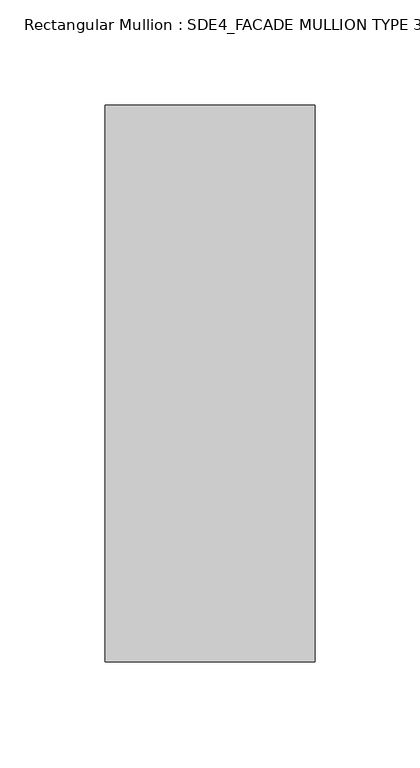
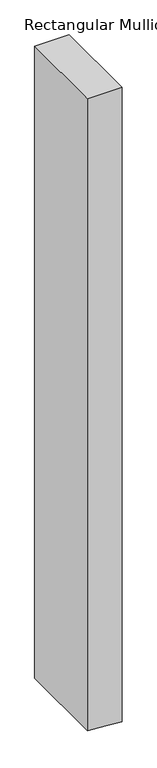
"""IFC4 building model written with IfcOpenShell, lengths in millimetres: member geometry, Rectangular Mullion : SDE4_FACADE MULLION TYPE 3."""

import ifcopenshell
import ifcopenshell.guid

model = None  # the IFC model being written
_history = None  # IfcOwnerHistory: only IFC2X3 demands one
_inside = {}  # id of a spatial element -> (the spatial element, [elements in it])
_under = {}  # id of a project, library or spatial element -> (it, [spatial elements below it])
_declared = {}  # id of a project -> (the project, [libraries it declares])
_typed = {}  # id of a type object -> (the type object, [elements of that type])
_made_of = {}  # id of a material, layer set ... -> (it, [elements and type objects made of it])


def new_model(schema):
    """Start an empty IFC model of exactly this schema.

    Asked for "IFC4X3", IfcOpenShell would pick the latest addendum, in which some entities
    have other attributes; the version numbers below select the first issue.
    IFC2X3 requires an IfcOwnerHistory on every rooted entity: one is made here for all.
    """
    global model, _history
    if schema == "IFC4X3":
        model = ifcopenshell.file(schema_version=(4, 3, 0, 0))
    else:
        model = ifcopenshell.file(schema=schema)
    _inside.clear()
    _under.clear()
    _declared.clear()
    _typed.clear()
    _made_of.clear()
    _history = None
    if model.schema == "IFC2X3":
        org = make("IfcOrganization", Name="unknown")
        user = make(
            "IfcPersonAndOrganization",
            ThePerson=make("IfcPerson", FamilyName="unknown"),
            TheOrganization=org,
        )
        app = make(
            "IfcApplication",
            ApplicationDeveloper=org,
            Version="unknown",
            ApplicationFullName="unknown",
            ApplicationIdentifier="unknown",
        )
        _history = make(
            "IfcOwnerHistory",
            OwningUser=user,
            OwningApplication=app,
            ChangeAction="ADDED",
            CreationDate=0,
        )
    return model


def make(cls, **values):
    """One entity of the class cls with the attributes given. An attribute that is None is left unset."""
    return model.create_entity(
        cls, **{name: value for name, value in values.items() if value is not None}
    )


def rooted(cls, **values):
    """An entity with a GlobalId (a new one), such as an element, a storey or a relation."""
    return make(cls, GlobalId=ifcopenshell.guid.new(), OwnerHistory=_history, **values)


def si_unit(unit_type, name, prefix=None):
    """IfcSIUnit, for example si_unit("LENGTHUNIT", "METRE", prefix="MILLI")."""
    return make("IfcSIUnit", UnitType=unit_type, Prefix=prefix, Name=name)


def assignment(units):
    """IfcUnitAssignment: the units of a project."""
    return None if units is None else make("IfcUnitAssignment", Units=units)


def point(xyz):
    """IfcCartesianPoint."""
    return None if xyz is None else make("IfcCartesianPoint", Coordinates=xyz)


def direction(xyz):
    """IfcDirection."""
    return None if xyz is None else make("IfcDirection", DirectionRatios=xyz)


def frame(location, z_axis=None, x_axis=None):
    """IfcAxis2Placement3D, a coordinate frame: its origin and axes. An axis left out is left unset."""
    return make(
        "IfcAxis2Placement3D",
        Location=point(location),
        Axis=direction(z_axis),
        RefDirection=direction(x_axis),
    )


def origin():
    """The frame at (0, 0, 0) with its axes left unset."""
    return frame((0.0, 0.0, 0.0))


def place(relative_to, where):
    """IfcLocalPlacement: puts the frame where relative to a parent placement (None: the world)."""
    return make(
        "IfcLocalPlacement", PlacementRelTo=relative_to, RelativePlacement=where
    )


def context(
    kind, dimensions, precision=None, world=None, true_north=None, identifier=None
):
    """IfcGeometricRepresentationContext, for example the 3D "Model" context."""
    return make(
        "IfcGeometricRepresentationContext",
        ContextIdentifier=identifier,
        ContextType=kind,
        CoordinateSpaceDimension=dimensions,
        Precision=precision,
        WorldCoordinateSystem=world,
        TrueNorth=true_north,
    )


def project(units=None, contexts=None):
    """IfcProject with its units and contexts."""
    return rooted(
        "IfcProject",
        Name="project",
        RepresentationContexts=contexts,
        UnitsInContext=assignment(units),
    )


def spatial(cls, under=None, at=None, **own):
    """A site, building, storey or space (cls), placed at a placement, below another one or the project."""
    s = rooted(cls, ObjectPlacement=at, **own)
    if under is not None:
        _under.setdefault(under.id(), (under, []))[1].append(s)
    return s


def polyline(points):
    """IfcPolyline through the points."""
    return make("IfcPolyline", Points=[point(p) for p in points])


def outline(outer, holes=None, kind="AREA"):
    """IfcArbitraryClosedProfileDef: a profile drawn as a closed curve; with holes, ...WithVoids."""
    if holes is None:
        return make("IfcArbitraryClosedProfileDef", ProfileType=kind, OuterCurve=outer)
    return make(
        "IfcArbitraryProfileDefWithVoids",
        ProfileType=kind,
        OuterCurve=outer,
        InnerCurves=holes,
    )


def extrude(swept, where, along, depth):
    """IfcExtrudedAreaSolid: the profile swept, set in the frame where, extruded along a direction by depth."""
    return make(
        "IfcExtrudedAreaSolid",
        SweptArea=swept,
        Position=where,
        ExtrudedDirection=direction(along),
        Depth=depth,
    )


def shape(context_of_items, identifier, shape_type, items):
    """IfcShapeRepresentation: the items that make up one representation, for example the "Body"."""
    return make(
        "IfcShapeRepresentation",
        ContextOfItems=context_of_items,
        RepresentationIdentifier=identifier,
        RepresentationType=shape_type,
        Items=items,
    )


def source(mapping_origin, context_of_items, identifier, shape_type, items):
    """IfcRepresentationMap: a shape defined once, which mapped items show again and again."""
    return make(
        "IfcRepresentationMap",
        MappingOrigin=mapping_origin,
        MappedRepresentation=shape(context_of_items, identifier, shape_type, items),
    )


def transform(
    local_origin,
    x_axis=None,
    y_axis=None,
    z_axis=None,
    scale=None,
    scale2=None,
    scale3=None,
    uniform=True,
):
    """IfcCartesianTransformationOperator3D, or its non-uniform kind. x_axis, y_axis, z_axis: its Axis1, 2, 3."""
    if uniform:
        return make(
            "IfcCartesianTransformationOperator3D",
            Axis1=direction(x_axis),
            Axis2=direction(y_axis),
            LocalOrigin=point(local_origin),
            Scale=scale,
            Axis3=direction(z_axis),
        )
    return make(
        "IfcCartesianTransformationOperator3DnonUniform",
        Axis1=direction(x_axis),
        Axis2=direction(y_axis),
        LocalOrigin=point(local_origin),
        Scale=scale,
        Axis3=direction(z_axis),
        Scale2=scale2,
        Scale3=scale3,
    )


def mapped(mapping_source, mapping_target):
    """IfcMappedItem: shows the shape of a source again, moved by a transform."""
    return make(
        "IfcMappedItem", MappingSource=mapping_source, MappingTarget=mapping_target
    )


def made_of(thing, what):
    """Note that an element or type object is made of a material, layer set ...; save() writes the relation."""
    if what is not None:
        _made_of.setdefault(what.id(), (what, []))[1].append(thing)
    return thing


def element(
    cls,
    number,
    at=None,
    inside=None,
    cuts=None,
    type_object=None,
    material=None,
    context=None,
    identifier="Body",
    shape_type=None,
    held_by="IfcProductDefinitionShape",
    body=None,
    shapes=None,
    **own,
):
    """One element of the class cls, such as IfcWall. Its Tag is "e" and its number.

    at: its placement. inside: the storey or other place that contains it. cuts: it is an
    opening in that element (IfcRelVoidsElement). A single representation is given by context,
    identifier, shape_type and body (its items); several are given by shapes. held_by: the class
    of the entity that holds the representations. save() writes the other relations.
    """
    e = rooted(cls, Tag="e%d" % number, ObjectPlacement=at, **own)
    if body is not None:
        shapes = [shape(context, identifier, shape_type, body)]
    if shapes is not None:
        e.Representation = make(held_by, Representations=shapes)
    if inside is not None:
        _inside.setdefault(inside.id(), (inside, []))[1].append(e)
    if cuts is not None:
        rooted(
            "IfcRelVoidsElement", RelatingBuildingElement=cuts, RelatedOpeningElement=e
        )
    if type_object is not None:
        _typed.setdefault(type_object.id(), (type_object, []))[1].append(e)
    return made_of(e, material)


def aggregate(whole, parts):
    """IfcRelAggregates: a whole, such as a stair, and the parts it consists of."""
    return rooted("IfcRelAggregates", RelatingObject=whole, RelatedObjects=parts)


def save(model, path):
    """Write the relations noted so far, then the file.

    IfcRelAggregates (storeys below a building ...), IfcRelContainedInSpatialStructure (elements
    in a storey), IfcRelDefinesByType, IfcRelAssociatesMaterial and IfcRelDeclares: one each for
    every whole, place, type object, material and project.
    """
    for whole, parts in _under.values():
        aggregate(whole, parts)
    for where, things in _inside.values():
        rooted(
            "IfcRelContainedInSpatialStructure",
            RelatedElements=things,
            RelatingStructure=where,
        )
    for kind, things in _typed.values():
        rooted("IfcRelDefinesByType", RelatedObjects=things, RelatingType=kind)
    for what, things in _made_of.values():
        rooted("IfcRelAssociatesMaterial", RelatedObjects=things, RelatingMaterial=what)
    for by, libraries in _declared.values():
        rooted("IfcRelDeclares", RelatingContext=by, RelatedDefinitions=libraries)
    model.write(path)


def rectangular_mullion_sde4_facade_mullion_type_3_e3ce9944(model_context):
    return source(origin(), model_context, "Body", "SweptSolid", [
        extrude(outline(polyline([(0.0, 50.0), (0.0, -50.0), (-1935.9007172, -50.0), (-1939.9667963, 3.056508), (-1943.5643936, 50.0), (0.0, 50.0)])), frame((0.0, -132.5, 0.0), z_axis=(0.0, 1.0, 0.0), x_axis=(0.0, 0.0, 1.0)), (0.0, 0.0, 1.0), 265.0),
    ])


if __name__ == "__main__":
    model = new_model("IFC4")
    model_context = context("Model", 3, world=origin())
    ifc_project = project(units=[si_unit("LENGTHUNIT", "METRE", prefix="MILLI")], contexts=[model_context])
    site = spatial("IfcSite", under=ifc_project)
    building = spatial("IfcBuilding", under=site)
    placement = place(None, origin())
    rectangular_mullion_sde4_facade_mullion_type_3_shape = rectangular_mullion_sde4_facade_mullion_type_3_e3ce9944(model_context)
    element("IfcMember", 1, ObjectType="Rectangular Mullion : SDE4_FACADE MULLION TYPE 3", at=placement, inside=building, context=model_context, shape_type="MappedRepresentation", body=[
        mapped(rectangular_mullion_sde4_facade_mullion_type_3_shape, transform((0.0, 0.0, 0.0), x_axis=(1.0, 0.0, 0.0), y_axis=(0.0, 1.0, 0.0), z_axis=(0.0, 0.0, 1.0))),
    ])
    save(model, "model.ifc")

# Revit data of these elements
# Type "Rectangular Mullion : SDE4_FACADE MULLION TYPE 3"
#   built-in parameter 1007322 = 0.869423 (stored number, unit not read)
#   built-in parameter 1007321 = 0.164042 (stored number, unit not read)
#   built-in parameter 1007320 = 0.164042 (stored number, unit not read)
